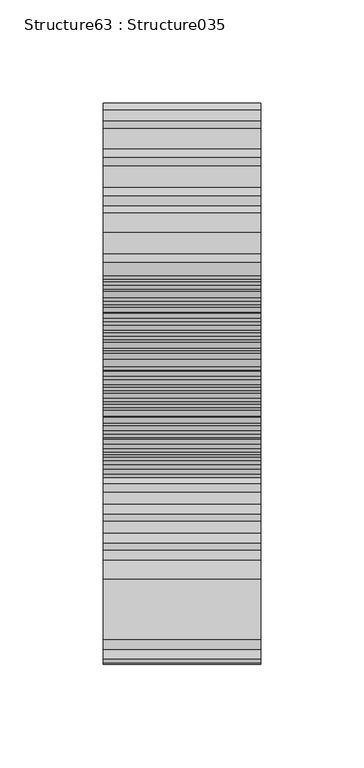
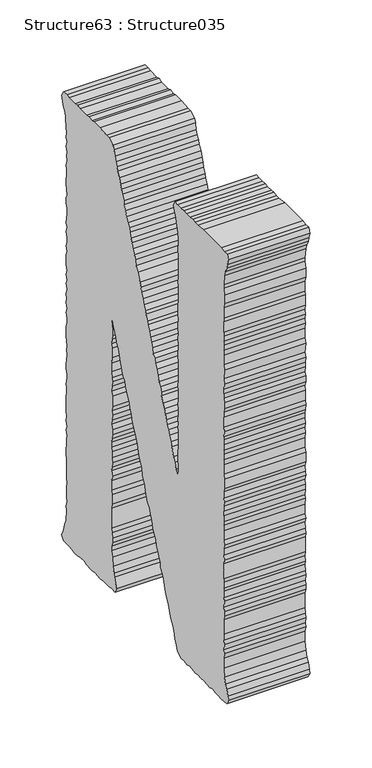
"""IFC4 building model written with IfcOpenShell, lengths in millimetres: proxy geometry, Structure63 : Structure035."""

from ifc_helpers import new_model, si_unit, frame, origin, place, context, project, spatial, polyline, outline, extrude, source, transform, mapped, element, save


def structure63_structure035_06d545ad(model_context):
    return source(origin(), model_context, "Body", "SweptSolid", [
        extrude(outline(polyline([(279034.0922984, 3575.0851816), (279035.2524274, 3583.2863152), (279036.4334164, 3589.1527492), (279036.4334164, 3593.8285667), (279035.2524274, 3597.9540049), (279035.2524274, 3602.0280957), (279035.8541541, 3607.3393366), (279036.4334164, 3611.4134274), (279036.4334164, 3631.3410106), (279035.8541541, 3635.4407751), (279035.8541541, 3644.8245022), (279036.4334164, 3648.9258713), (279036.4334164, 3658.3015753), (279035.2524274, 3663.5598643), (279036.4334164, 3668.2437048), (279035.8541541, 3672.3691429), (279035.2524274, 3677.0449604), (279035.8541541, 3681.7271964), (279035.8541541, 3687.587212), (279036.4334164, 3691.6869765), (279036.4334164, 3696.3884676), (279035.8541541, 3700.4705815), (279035.2524274, 3704.5879966), (279035.2524274, 3709.8559132), (279036.4334164, 3714.5301261), (279035.8541541, 3718.6571688), (279035.2524274, 3723.9154578), (279035.8541541, 3728.0152223), (279035.2524274, 3732.7167134), (279035.2524274, 3742.6748889), (279036.4334164, 3747.3587295), (279035.8541541, 3752.6170184), (279035.2524274, 3757.3185096), (279035.8541541, 3760.818152), (279036.4334164, 3766.684586), (279036.4334164, 3774.8857196), (279035.8541541, 3780.7441306), (279035.8541541, 3790.1294623), (279036.4334164, 3794.2292268), (279035.8541541, 3798.9050443), (279035.2524274, 3803.0064134), (279035.2524274, 3808.8888934), (279035.8541541, 3812.9726119), (279036.4334164, 3818.2309008), (279035.2524274, 3817.6741031), (279032.9113095, 3812.9726119), (279031.1510584, 3808.290376), (279029.4132717, 3804.7730829), (279028.2322828, 3800.6717138), (279025.3119026, 3795.960595), (279023.529187, 3790.7039107), (279022.3706626, 3787.2042683), (279021.1896736, 3782.5027771), (279019.4294225, 3777.8285642), (279017.6900312, 3773.7015215), (279014.7487912, 3770.2018791), (279013.5902668, 3766.1021146), (279011.2491488, 3760.2437036), (279010.0681599, 3757.3185096), (279007.7286465, 3752.6170184), (279006.5476576, 3748.5429276), (279004.2065397, 3743.8414364), (279003.6272774, 3739.1592005), (279000.7085019, 3733.8736333), (278999.527513, 3730.3563402), (278997.1655351, 3725.6741043), (278995.4261439, 3722.1568112), (278993.6658927, 3716.8985223), (278993.0866305, 3712.7971532), (278991.3263794, 3708.087639), (278988.9852614, 3703.4134261), (278987.2250103, 3700.4705815), (278986.0440214, 3694.6298211), (278984.2837702, 3691.0868544), (278981.9426523, 3686.4030139), (278981.3633901, 3681.7271964), (278977.8428878, 3672.9435914), (278974.9016478, 3668.8261762), (278973.1622565, 3664.1423357), (278971.9812676, 3660.6250426), (278969.6417542, 3655.9428067), (278969.062492, 3651.8590883), (278966.721374, 3647.1575971), (278964.3593962, 3643.6579547), (278963.780134, 3638.3563415), (278961.4406206, 3634.2822506), (278959.6787649, 3630.1824862), (278957.3392516, 3625.472972), (278956.7375249, 3621.3732075), (278953.8187493, 3616.69739), (278952.0568936, 3613.1720739), (278950.2966424, 3607.3393366), (278949.7173802, 3603.7963698), (278947.9571291, 3599.7126514), (278944.4350222, 3591.5131224), (278942.0955088, 3586.8116312), (278940.9145199, 3581.5276686), (278938.5750066, 3577.4535778), (278936.2338886, 3573.3265351), (278934.4736375, 3568.0682461), (278933.8943753, 3563.9412034), (278930.9755997, 3559.2669905), (278929.213744, 3555.1848766), (278923.3537283, 3551.0658569), (278919.2523592, 3551.0658569), (278913.9700012, 3550.4833855), (278909.2909745, 3551.6675836), (278905.7688677, 3551.6675836), (278900.4881143, 3550.4833855), (278895.807483, 3551.6675836), (278891.7061139, 3550.4833855), (278885.8460983, 3551.0658569), (278882.3464558, 3551.0658569), (278876.4848356, 3550.4833855), (278872.9643334, 3551.6675836), (278867.6819754, 3551.0658569), (278863.5822109, 3551.0658569), (278857.7430551, 3550.4833855), (278853.6192216, 3551.0658569), (278849.5194571, 3551.0658569), (278846.0198147, 3556.3417965), (278847.1783391, 3559.8671125), (278848.9401949, 3565.7094775), (278851.2797082, 3569.2524442), (278853.0399593, 3575.0851816), (278854.2209482, 3583.2863152), (278854.2209482, 3593.2541183), (278853.0399593, 3598.5284533), (278853.6192216, 3602.0280957), (278853.0399593, 3607.3393366), (278853.6192216, 3611.4134274), (278854.2209482, 3616.69739), (278854.2209482, 3631.3410106), (278853.0399593, 3635.4407751), (278853.0399593, 3640.114988), (278853.6192216, 3644.2420307), (278853.0399593, 3650.1004418), (278853.6192216, 3653.6000842), (278854.2209482, 3659.4584952), (278853.6192216, 3662.9854159), (278854.2209482, 3668.2437048), (278853.6192216, 3672.3691429), (278853.6192216, 3687.0127636), (278853.0399593, 3691.0868544), (278853.6192216, 3695.786741), (278854.2209482, 3701.6547796), (278853.0399593, 3705.7545441), (278854.2209482, 3709.8559132), (278854.2209482, 3719.2316172), (278853.6192216, 3725.0996559), (278854.2209482, 3728.5992983), (278853.6192216, 3734.47536), (278853.6192216, 3739.1592005), (278854.2209482, 3743.8414364), (278853.0399593, 3748.5429276), (278853.6192216, 3752.04257), (278854.2209482, 3757.8753073), (278853.0399593, 3762.0023501), (278853.0399593, 3771.3860772), (278854.2209482, 3775.4874463), (278854.2209482, 3784.8438951), (278853.6192216, 3790.1294623), (278854.2209482, 3795.4037973), (278853.6192216, 3799.5051664), (278854.2209482, 3804.7730829), (278854.2209482, 3809.4729695), (278853.6192216, 3812.9726119), (278853.0399593, 3818.2309008), (278853.6192216, 3822.348316), (278853.6192216, 3832.3161191), (278854.2209482, 3836.9919366), (278853.0399593, 3841.0900965), (278853.0399593, 3846.9757858), (278854.2209482, 3850.4754282), (278853.6192216, 3855.7353217), (278853.6192216, 3859.8591552), (278853.0399593, 3865.1190488), (278854.2209482, 3869.8189354), (278853.0399593, 3879.1769888), (278854.2209482, 3883.8881076), (278854.2209482, 3893.246161), (278853.6192216, 3898.5301236), (278854.2209482, 3903.2059411), (278853.6192216, 3907.3313793), (278854.2209482, 3912.0071968), (278853.6192216, 3916.6653636), (278853.6192216, 3926.6492128), (278854.2209482, 3930.1745289), (278854.2209482, 3940.1166583), (278853.0399593, 3944.8165449), (278853.0399593, 3953.5937315), (278854.2209482, 3959.4617701), (278854.2209482, 3962.9774586), (278853.0399593, 3972.9372387), (278851.2797082, 3977.6194746), (278848.9401949, 3982.8793681), (278848.359328, 3986.4046842), (278846.5990769, 3992.2614906), (278848.359328, 3996.9645864), (278853.0399593, 3996.390138), (278857.7430551, 3997.5486624), (278887.0270872, 3997.5486624), (278896.3867452, 3996.390138), (278901.089841, 3996.390138), (278904.6103432, 3997.5486624), (278909.2909745, 3996.390138), (278915.1509902, 3996.390138), (278918.6506326, 3997.5486624), (278923.3537283, 3996.9645864), (278929.213744, 3996.9645864), (278933.315113, 3997.5486624), (278936.2338886, 3992.2614906), (278934.4736375, 3987.5792547), (278932.1341241, 3982.3225704), (278930.9755997, 3978.2035506), (278929.213744, 3972.9372387), (278927.4534928, 3964.1343784), (278927.4534928, 3959.4617701), (278928.6344817, 3954.7506513), (278927.4534928, 3944.235678), (278928.032755, 3940.718385), (278927.4534928, 3936.0345445), (278928.032755, 3930.7329312), (278928.032755, 3925.4746423), (278928.6344817, 3921.3748778), (278927.4534928, 3916.6653636), (278928.032755, 3912.5896682), (278928.032755, 3903.2059411), (278928.6344817, 3897.3475301), (278928.6344817, 3887.9621984), (278927.4534928, 3884.4609514), (278928.6344817, 3878.5784713), (278928.6344817, 3873.9203044), (278928.032755, 3870.4030114), (278928.6344817, 3864.5446004), (278927.4534928, 3859.8591552), (278927.4534928, 3856.3161885), (278928.6344817, 3850.4754282), (278928.6344817, 3846.9757858), (278927.4534928, 3842.2758992), (278927.4534928, 3832.8921721), (278928.032755, 3828.2163546), (278927.4534928, 3823.5341187), (278928.6344817, 3818.2309008), (278928.032755, 3813.5743386), (278927.4534928, 3810.0474179), (278928.032755, 3804.1890069), (278928.6344817, 3800.0876378), (278927.4534928, 3794.8309535), (278927.4534928, 3790.1294623), (278928.6344817, 3785.4456218), (278927.4534928, 3780.7441306), (278928.6344817, 3777.2444882), (278928.032755, 3772.5606477), (278928.032755, 3767.2590344), (278927.4534928, 3762.5848215), (278927.4534928, 3757.3185096), (278928.6344817, 3753.8012165), (278928.6344817, 3744.4158848), (278927.4534928, 3738.5574738), (278927.4534928, 3735.0578314), (278928.6344817, 3730.3563402), (278929.7930062, 3729.1737467), (278931.5548619, 3733.2991849), (278933.8943753, 3739.1592005), (278935.6546264, 3743.2332913), (278937.9957444, 3752.04257), (278940.3577222, 3755.559863), (278942.6972355, 3760.2437036), (278944.4350222, 3764.9435901), (278946.1968779, 3768.4432325), (278947.3778668, 3773.11905), (278948.5363913, 3777.8285642), (278950.2966424, 3781.9299333), (278952.6377604, 3786.0280932), (278954.9997382, 3791.8865042), (278955.5790004, 3795.4037973), (278957.3392516, 3799.5051664), (278959.0995027, 3803.5872802), (278961.4406206, 3808.290376), (278962.6216096, 3813.5743386), (278965.5403851, 3817.6741031), (278966.1196474, 3822.348316), (278969.062492, 3825.2911606), (278970.2210164, 3830.5574726), (278971.9812676, 3834.6588416), (278973.1622565, 3838.7586061), (278974.9016478, 3844.0345457), (278977.2636256, 3848.7167816), (278978.42215, 3851.6612309), (278980.1824012, 3857.5019912), (278981.3633901, 3860.4432313), (278983.704508, 3864.5446004), (278985.4647592, 3869.8189354), (278987.8042725, 3874.5043805), (278988.3835347, 3879.1769888), (278990.1453905, 3883.2863809), (278993.6658927, 3890.905043), (278996.5846683, 3895.5888836), (278997.7672618, 3900.8648231), (278998.9257863, 3904.9645876), (279001.8670263, 3909.0627475), (279003.0480152, 3914.3499193), (279004.7874065, 3917.8479571), (279006.5476576, 3922.5494483), (279007.7286465, 3926.6492128), (279010.0681599, 3930.1745289), (279011.828411, 3934.8503464), (279013.5902668, 3939.5325823), (279015.9297801, 3944.235678), (279016.5090423, 3947.7337158), (279018.8485557, 3952.9920048), (279020.0311492, 3957.1190475), (279021.7914003, 3961.2204166), (279023.529187, 3966.5043792), (279026.470427, 3971.1785921), (279027.6530206, 3974.7055128), (279029.4132717, 3978.8036727), (279031.1510584, 3982.8793681), (279032.3320473, 3988.7634528), (279034.0922984, 3992.2614906), (279040.5331808, 3995.7803883), (279044.6345499, 3995.7803883), (279055.1751969, 3996.9645864), (279064.558924, 3996.9645864), (279068.0794262, 3995.7803883), (279072.7600575, 3996.9645864), (279076.859822, 3995.7803883), (279087.4020736, 3995.7803883), (279091.501838, 3996.9645864), (279095.6032071, 3995.7803883), (279105.5870563, 3995.7803883), (279109.0866987, 3996.9645864), (279114.3674521, 3996.390138), (279117.8670945, 3991.0788971), (279116.1277032, 3986.4046842), (279114.9467143, 3982.8793681), (279112.0279388, 3977.6194746), (279110.8469498, 3973.5197101), (279110.2676876, 3962.9774586), (279109.6659609, 3959.4617701), (279110.2676876, 3953.5937315), (279109.0866987, 3950.0940891), (279110.2676876, 3944.8165449), (279109.0866987, 3940.1166583), (279109.6659609, 3936.0345445), (279109.0866987, 3931.3346579), (279110.2676876, 3926.6492128), (279109.6659609, 3921.9733953), (279109.6659609, 3916.0909152), (279110.2676876, 3912.5896682), (279110.2676876, 3907.3313793), (279109.6659609, 3902.6314927), (279109.0866987, 3897.3475301), (279110.2676876, 3893.822214), (279110.2676876, 3888.5623205), (279109.0866987, 3884.4609514), (279109.0866987, 3879.1769888), (279109.6659609, 3873.9203044), (279110.2676876, 3869.2444869), (279109.0866987, 3865.7015202), (279110.2676876, 3861.0192843), (279109.0866987, 3855.1769193), (279109.0866987, 3851.0595042), (279110.2676876, 3846.3772683), (279109.0866987, 3841.6741725), (279110.2676876, 3837.6000817), (279110.2676876, 3828.2163546), (279109.0866987, 3822.348316), (279110.2676876, 3818.2309008), (279109.0866987, 3812.9726119), (279110.2676876, 3809.4729695), (279109.0866987, 3804.1890069), (279110.2676876, 3798.9050443), (279109.6659609, 3794.2292268), (279110.2676876, 3790.7039107), (279109.0866987, 3784.8438951), (279110.2676876, 3780.7441306), (279109.0866987, 3776.0618947), (279109.0866987, 3771.3860772), (279110.2676876, 3766.684586), (279110.2676876, 3757.3185096), (279109.6659609, 3752.04257), (279109.0866987, 3747.9428055), (279109.6659609, 3743.8414364), (279109.0866987, 3739.1592005), (279109.6659609, 3733.8736333), (279110.2676876, 3729.7738688), (279110.2676876, 3725.0996559), (279109.0866987, 3719.2316172), (279109.0866987, 3715.7143242), (279110.2676876, 3709.8559132), (279109.6659609, 3706.3289925), (279109.6659609, 3701.6547796), (279110.2676876, 3696.9709391), (279110.2676876, 3682.3289231), (279109.6659609, 3678.2018803), (279110.2676876, 3672.9435914), (279109.0866987, 3667.6853024), (279110.2676876, 3664.1423357), (279109.0866987, 3659.4584952), (279109.6659609, 3654.7842823), (279109.6659609, 3649.5003197), (279110.2676876, 3644.8245022), (279110.2676876, 3640.114988), (279109.6659609, 3635.4407751), (279109.6659609, 3616.69739), (279109.0866987, 3612.0135494), (279109.6659609, 3607.8961343), (279109.6659609, 3597.9540049), (279109.0866987, 3593.2541183), (279110.2676876, 3589.1527492), (279109.6659609, 3584.4689087), (279110.2676876, 3574.5107332), (279112.607201, 3569.2524442), (279113.7657254, 3565.1254015), (279114.9467143, 3561.025637), (279117.8670945, 3555.7416744), (279114.3674521, 3551.6675836), (279104.9853296, 3551.6675836), (279095.6032071, 3550.4833855), (279090.9225758, 3550.4833855), (279087.4020736, 3551.6675836), (279081.5404533, 3551.6675836), (279077.4390842, 3550.4833855), (279068.6586884, 3550.4833855), (279063.3987949, 3551.0658569), (279059.276566, 3550.4833855), (279054.0166724, 3550.4833855), (279050.4961702, 3551.0658569), (279040.5331808, 3551.0658569), (279035.8541541, 3551.6675836), (279031.1510584, 3551.0658569), (279028.2322828, 3556.3417965), (279031.752785, 3565.7094775), (279032.3320473, 3569.2524442), (279034.0922984, 3575.0851816)])), frame((-59031.6926606, 0.0, 0.0), z_axis=(1.0, 0.0, 0.0), x_axis=(0.0, 1.0, 0.0)), (0.0, 0.0, 1.0), 76.2),
    ])


if __name__ == "__main__":
    model = new_model("IFC4")
    model_context = context("Model", 3, world=origin())
    ifc_project = project(units=[si_unit("LENGTHUNIT", "METRE", prefix="MILLI")], contexts=[model_context])
    site = spatial("IfcSite", under=ifc_project)
    building = spatial("IfcBuilding", under=site)
    placement = place(None, origin())
    structure63_structure035_shape = structure63_structure035_06d545ad(model_context)
    element("IfcBuildingElementProxy", 1, Name="Structure63 : Structure035", ObjectType="Structure63 : Structure035", at=placement, inside=building, context=model_context, shape_type="MappedRepresentation", body=[
        mapped(structure63_structure035_shape, transform((0.0, 0.0, 0.0), x_axis=(1.0, 0.0, 0.0), y_axis=(0.0, 1.0, 0.0), z_axis=(0.0, 0.0, 1.0))),
    ])
    save(model, "model.ifc")

# Revit data of these elements
# Type "Structure63 : Structure035"
#   NameOverride = "Structure035"
# Element 1 (IfcBuildingElementProxy, "Structure63 : Structure035")
#   Materials on its faces: "BRUSHED ALUM. LETTERING"
# Materials
#   "BRUSHED ALUM. LETTERING": class "Unassigned", colour RGB 169 181 186, transparency 0, Cost = 0
